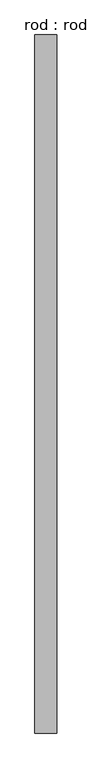
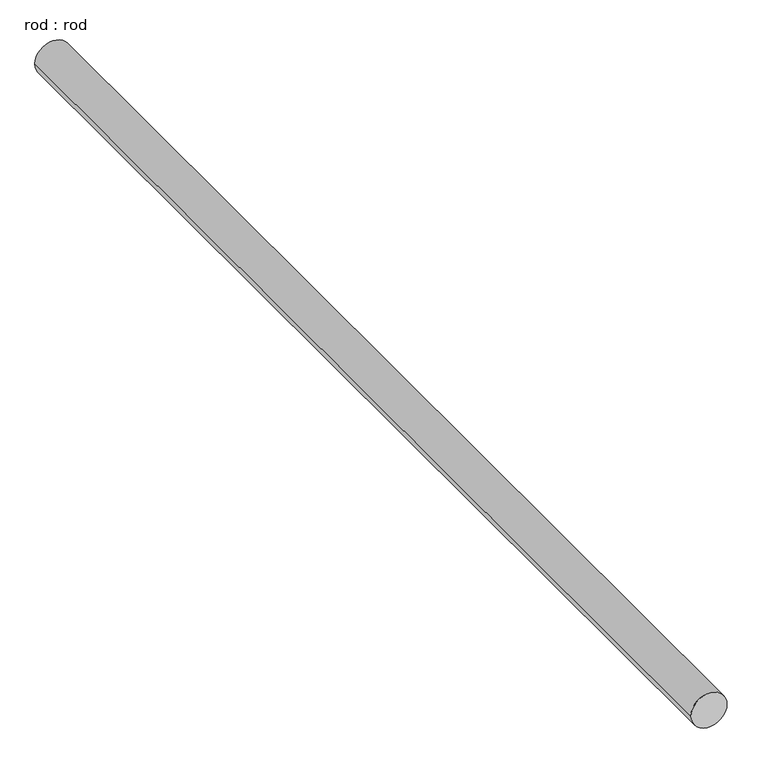
"""IFC4 building model written with IfcOpenShell, lengths in millimetres: proxy geometry, rod : rod."""

from ifc_helpers import new_model, si_unit, point, frame, frame_2d, origin, place, context, project, spatial, circle_curve, trimmed, segment, composite_curve, outline, extrude, source, transform, mapped, element, save


def rod_rod_67e8fedd(model_context):
    return source(origin(), model_context, "Body", "SweptSolid", [
        extrude(outline(composite_curve([segment(trimmed(circle_curve(frame_2d((0.0108462, 0.0)), 200.0), [point((0.0108462, 200.0))], [point((0.0108462, -200.0))], False, "CARTESIAN"), True, "CONTINUOUS"), segment(trimmed(circle_curve(frame_2d((0.0108462, 0.0)), 200.0), [point((0.0108462, -200.0))], [point((0.0108462, 200.0))], False, "CARTESIAN"), True, "CONTINUOUS")], self_intersect=False)), frame((0.0, -2235.308326, 0.0), z_axis=(0.0, 1.0, 0.0), x_axis=(0.0, 0.0, 1.0)), (0.0, 0.0, 1.0), 12656.0738826),
    ])


if __name__ == "__main__":
    model = new_model("IFC4")
    model_context = context("Model", 3, world=origin())
    ifc_project = project(units=[si_unit("LENGTHUNIT", "METRE", prefix="MILLI")], contexts=[model_context])
    site = spatial("IfcSite", under=ifc_project)
    building = spatial("IfcBuilding", under=site)
    placement = place(None, origin())
    rod_rod_shape = rod_rod_67e8fedd(model_context)
    element("IfcBuildingElementProxy", 1, Name="rod : rod", ObjectType="rod : rod", at=placement, inside=building, context=model_context, shape_type="MappedRepresentation", body=[
        mapped(rod_rod_shape, transform((0.0, 0.0, 0.0), x_axis=(1.0, 0.0, 0.0), y_axis=(0.0, 1.0, 0.0), z_axis=(0.0, 0.0, 1.0))),
    ])
    save(model, "model.ifc")

# Revit data of these elements
# Type "rod : rod"
#   Default Elevation = 0
